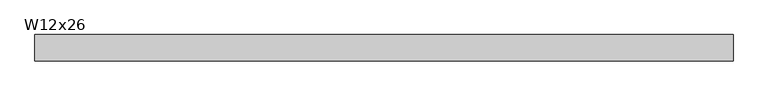
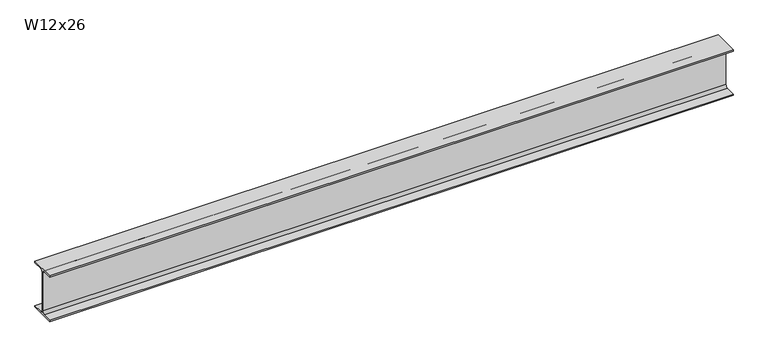
"""IFC4 building model written with IfcOpenShell, lengths in millimetres: beam geometry, RME W-Wide Flange : W12x26."""

from ifc_helpers import new_model, si_unit, point, frame, frame_2d, origin, place, context, project, spatial, polyline, circle_curve, trimmed, segment, composite_curve, outline, extrude, source, transform, mapped, element, save


def w12x26_79a0c7f6(model_context):
    return source(origin(), model_context, "Body", "SweptSolid", [
        extrude(outline(composite_curve([segment(polyline([(82.423, -145.288), (82.423, -154.94), (-82.423, -154.94), (-82.423, -145.288), (-20.2565, -145.288)]), True, "CONTINUOUS"), segment(trimmed(circle_curve(frame_2d((-20.2565, -127.9525)), 17.3355), [point((-20.2565, -145.288))], [point((-2.921, -127.9525))], True, "CARTESIAN"), True, "CONTINUOUS"), segment(polyline([(-2.921, -127.9525), (-2.921, 127.9525)]), True, "CONTINUOUS"), segment(trimmed(circle_curve(frame_2d((-20.2565, 127.9525)), 17.3355), [point((-2.921, 127.9525))], [point((-20.2565, 145.288))], True, "CARTESIAN"), True, "CONTINUOUS"), segment(polyline([(-20.2565, 145.288), (-82.423, 145.288), (-82.423, 154.94), (82.423, 154.94), (82.423, 145.288), (20.2565, 145.288)]), True, "CONTINUOUS"), segment(trimmed(circle_curve(frame_2d((20.2565, 127.9525)), 17.3355), [point((20.2565, 145.288))], [point((2.921, 127.9525))], True, "CARTESIAN"), True, "CONTINUOUS"), segment(polyline([(2.921, 127.9525), (2.921, -127.9525)]), True, "CONTINUOUS"), segment(trimmed(circle_curve(frame_2d((20.2565, -127.9525)), 17.3355), [point((2.921, -127.9525))], [point((20.2565, -145.288))], True, "CARTESIAN"), True, "CONTINUOUS"), segment(polyline([(20.2565, -145.288), (82.423, -145.288)]), True, "CONTINUOUS")], self_intersect=False)), frame((-2253.996, 0.0, 0.0), z_axis=(1.0, 0.0, 0.0), x_axis=(0.0, 1.0, 0.0)), (0.0, 0.0, 1.0), 4372.7796786),
    ])


if __name__ == "__main__":
    model = new_model("IFC4")
    model_context = context("Model", 3, world=origin())
    ifc_project = project(units=[si_unit("LENGTHUNIT", "METRE", prefix="MILLI")], contexts=[model_context])
    site = spatial("IfcSite", under=ifc_project)
    building = spatial("IfcBuilding", under=site)
    placement = place(None, origin())
    w12x26_shape = w12x26_79a0c7f6(model_context)
    element("IfcBeam", 1, ObjectType="RME W-Wide Flange : W12x26", at=placement, inside=building, context=model_context, shape_type="MappedRepresentation", body=[
        mapped(w12x26_shape, transform((0.0, 0.0, 0.0), x_axis=(1.0, 0.0, 0.0), y_axis=(0.0, 1.0, 0.0), z_axis=(0.0, 0.0, 1.0))),
    ])
    save(model, "model.ifc")

# Revit data of these elements
# Type "RME W-Wide Flange : W12x26"
#   WELD P [instance default] = ""
#   WELD LE [instance default] = ""
#   WELD D [instance default] = ""
#   TOP SECTION SIZE [instance default] = ""
#   TOP SECTION LENGTH [instance default] = ""
#   REMARKS [instance default] = ""
#   REINF TYPE [instance default] = ""
#   Nominal Size = "W24"
#   End Bearing Capacity [instance default] = ""
#   BOT SECTION SIZE [instance default] = ""
#   BOT SECTION LENGTH [instance default] = ""
#   Assembly Code = "B10"
#   W = 26
#   Start Extension Calculation [instance default] = 10' - 0"
#   Start Extension [instance default] = -0' - 0 1/2"
#   End Extension Calculation [instance default] = 10' - 0"
#   End Extension [instance default] = -0' - 0 1/2"
#   Length [instance default] = 5' - 0"
#   bf = 0' - 6.49"
#   d = 1' - 0.2"
#   k = 0' - 1 1/16"
#   k2 = 0' - 0.6825"
#   tf = 0' - 0.38"
#   tw = 0' - 0.23"
#   A = 0.053125 SF
#   Structural Material [instance default] = Metal - Steel - ASTM A992
# Element 1 (IfcBeam, "RME W-Wide Flange : W12x26")
#   End Extension Calculation = 12' - 0.82543"
#   End Extension = 2' - 0.32543"
#   Length = 14' - 9.48"
#   Materials on its faces: "Metal - Steel - ASTM A992"
# Materials
#   "Metal - Steel - ASTM A992": class "Metal", colour RGB 255 128 0, transparency 0
